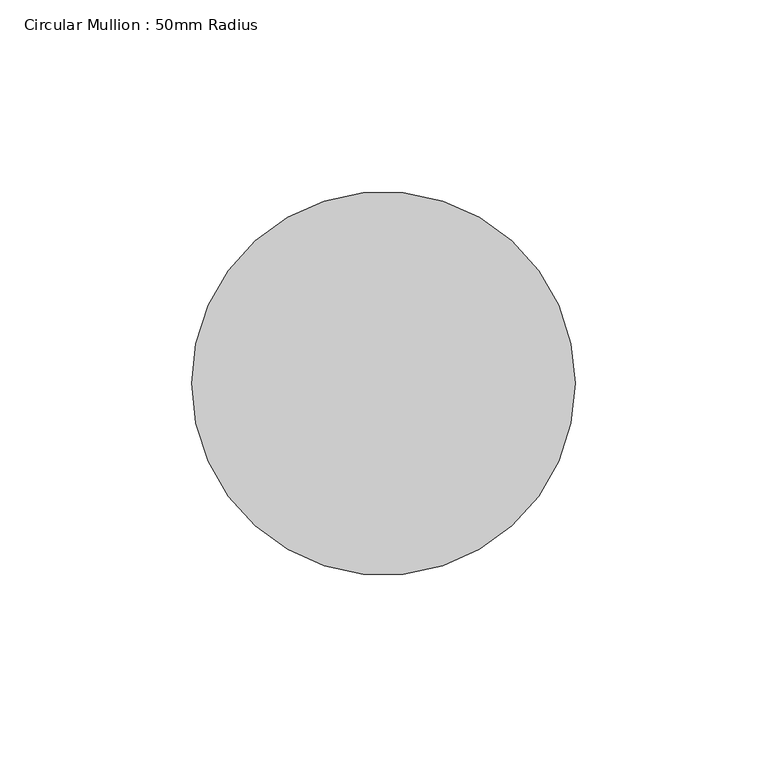
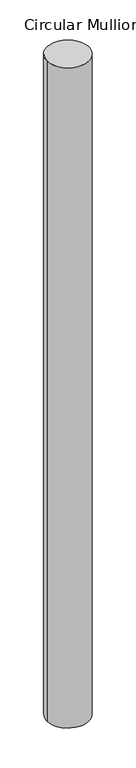
"""IFC4 building model written with IfcOpenShell, lengths in millimetres: member geometry, Circular Mullion : 50mm Radius."""

from ifc_helpers import new_model, si_unit, point, frame, origin, origin_2d, place, context, project, spatial, circle_curve, trimmed, segment, composite_curve, outline, extrude, source, transform, mapped, element, save


def circular_mullion_50mm_radius_6b8c3653(model_context):
    return source(origin(), model_context, "Body", "SweptSolid", [
        extrude(outline(composite_curve([segment(trimmed(circle_curve(origin_2d(), 50.0), [point((50.0, 0.0))], [point((-50.0, 0.0))], False, "CARTESIAN"), True, "CONTINUOUS"), segment(trimmed(circle_curve(origin_2d(), 50.0), [point((-50.0, 0.0))], [point((50.0, 0.0))], False, "CARTESIAN"), True, "CONTINUOUS")], self_intersect=False)), frame((0.0, 0.0, -1660.2882413), z_axis=(0.0, 0.0, 1.0), x_axis=(1.0, 0.0, 0.0)), (0.0, 0.0, 1.0), 1660.2882413),
    ])


if __name__ == "__main__":
    model = new_model("IFC4")
    model_context = context("Model", 3, world=origin())
    ifc_project = project(units=[si_unit("LENGTHUNIT", "METRE", prefix="MILLI")], contexts=[model_context])
    site = spatial("IfcSite", under=ifc_project)
    building = spatial("IfcBuilding", under=site)
    placement = place(None, origin())
    circular_mullion_50mm_radius_shape = circular_mullion_50mm_radius_6b8c3653(model_context)
    element("IfcMember", 1, ObjectType="Circular Mullion : 50mm Radius", at=placement, inside=building, context=model_context, shape_type="MappedRepresentation", body=[
        mapped(circular_mullion_50mm_radius_shape, transform((0.0, 0.0, 0.0), x_axis=(1.0, 0.0, 0.0), y_axis=(0.0, 1.0, 0.0), z_axis=(0.0, 0.0, 1.0))),
    ])
    save(model, "model.ifc")

# Revit data of these elements
# Type "Circular Mullion : 50mm Radius"
#   built-in parameter 1007350 = 0.164042 (stored number, unit not read)
# Element 1 (IfcMember, "Circular Mullion : 50mm Radius")
#   Materials on its faces: "Aluminium"
# Materials
#   "Aluminium": class "Metal", colour RGB 247 247 247, transparency 0, Description = "Aluminium 6061", Cost = 0
